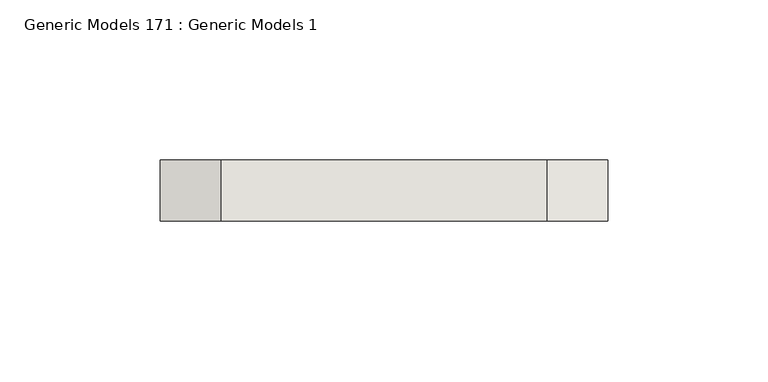
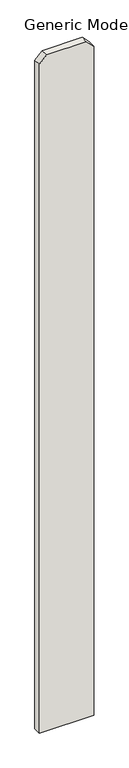
"""IFC4 building model written with IfcOpenShell, lengths in millimetres: wall geometry, Generic Models 171 : Generic Models 1."""

from ifc_helpers import new_model, si_unit, frame, origin, place, context, project, spatial, polyline, outline, extrude, source, transform, mapped, element, save


def generic_models_171_generic_models_1_02e9bb0c(model_context):
    return source(origin(), model_context, "Body", "SweptSolid", [
        extrude(outline(polyline([(76.2, 325042.2125), (1885.95, 325042.2125), (1905.0, 325023.1625), (1905.0, 324921.5625), (1885.95, 324902.5125), (76.2, 324902.5125), (76.2, 325042.2125)])), frame((0.0, 547.6875, 0.0), z_axis=(0.0, 1.0, 0.0), x_axis=(0.0, 0.0, 1.0)), (0.0, 0.0, 1.0), 19.05),
    ])


if __name__ == "__main__":
    model = new_model("IFC4")
    model_context = context("Model", 3, world=origin())
    ifc_project = project(units=[si_unit("LENGTHUNIT", "METRE", prefix="MILLI")], contexts=[model_context])
    site = spatial("IfcSite", under=ifc_project)
    building = spatial("IfcBuilding", under=site)
    placement = place(None, origin())
    generic_models_171_generic_models_1_shape = generic_models_171_generic_models_1_02e9bb0c(model_context)
    element("IfcWall", 1, ObjectType="Generic Models 171 : Generic Models 1", at=placement, inside=building, context=model_context, shape_type="MappedRepresentation", body=[
        mapped(generic_models_171_generic_models_1_shape, transform((0.0, 0.0, 0.0), x_axis=(1.0, 0.0, 0.0), y_axis=(0.0, 1.0, 0.0), z_axis=(0.0, 0.0, 1.0))),
    ])
    save(model, "model.ifc")

# Revit data of these elements
# Element 1 (IfcWall, "Generic Models 171 : Generic Models 1")
#   Materials on its faces: "VERTICAL 1X6 CEDAR PLANKS W/ CLEAR WOOD SEALER"
# Materials
#   "VERTICAL 1X6 CEDAR PLANKS W/ CLEAR WOOD SEALER": class "Wood", colour RGB 234 198 147, transparency 0, Description = "Pinus Echinata", Cost = 0
